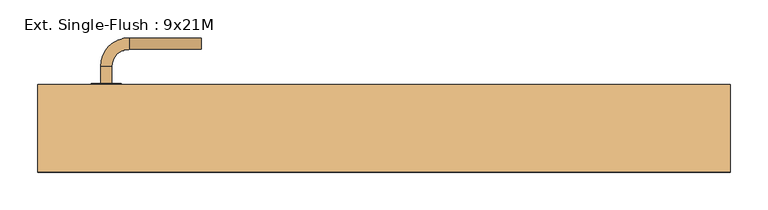
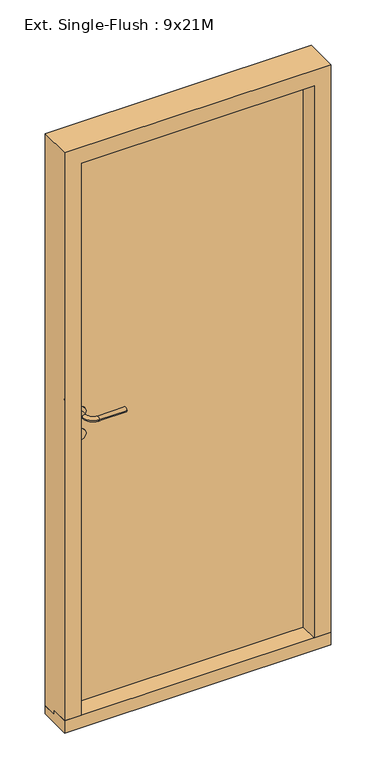
"""IFC4 building model written with IfcOpenShell, lengths in millimetres: door geometry, Ext. Single-Flush : 9x21M."""

from ifc_helpers import new_model, si_unit, point, frame, frame_2d, origin, place, context, project, spatial, polyline, circle_curve, ellipse_curve, trimmed, segment, composite_curve, outline, extrude, faceted_brep, source, transform, mapped, element, save
from ifc_brep_helpers import plane_surface, cylinder_surface, revolved_surface, advanced_brep


def ext_single_flush_9x21m_44480e6f(model_context):
    return source(origin(), model_context, "Body", "SolidModel", [
        extrude(outline(composite_curve([segment(trimmed(circle_curve(frame_2d((1090.0, -366.0)), 20.0), [point((1070.0, -366.0))], [point((1110.0, -366.0))], False, "CARTESIAN"), True, "CONTINUOUS"), segment(trimmed(circle_curve(frame_2d((1090.0, -366.0)), 20.0), [point((1110.0, -366.0))], [point((1070.0, -366.0))], False, "CARTESIAN"), True, "CONTINUOUS")], self_intersect=False)), frame((0.0, 184.0, 0.0), z_axis=(0.0, 1.0, 0.0), x_axis=(0.0, 0.0, 1.0)), (0.0, 0.0, 1.0), 2.0),
        advanced_brep(
        [(-373.5, 186.0, 1090.0), (-358.5, 186.0, 1090.0), (-373.5, 208.5, 1090.0), (-358.5, 208.5, 1090.0), (-336.0, 231.0, 1090.0), (-336.0, 246.0, 1090.0), (-241.0, 246.0, 1090.0), (-241.0, 231.0, 1090.0)],
        [
            (0, 1, circle_curve(frame((-366.0, 186.0, 1090.0), z_axis=(0.0, -1.0, 0.0), x_axis=(1.0, 0.0, 0.0)), 7.5)),
            (1, 0, circle_curve(frame((-366.0, 186.0, 1090.0), z_axis=(0.0, -1.0, 0.0), x_axis=(1.0, 0.0, 0.0)), 7.5)),
            (0, 2),
            (2, 3, circle_curve(frame((-366.0, 208.5, 1090.0), z_axis=(0.0, -1.0, 0.0), x_axis=(1.0, 0.0, 0.0)), 7.5)),
            (3, 1),
            (3, 2, circle_curve(frame((-366.0, 208.5, 1090.0), z_axis=(0.0, -1.0, 0.0), x_axis=(1.0, 0.0, 0.0)), 7.5)),
            (4, 3, circle_curve(frame((-336.0, 208.5, 1090.0), z_axis=(0.0, 0.0, 1.0), x_axis=(-1.0, 0.0, 0.0)), 22.5)),
            (2, 5, circle_curve(frame((-336.0, 208.5, 1090.0), z_axis=(0.0, 0.0, -1.0), x_axis=(-1.0, 0.0, 0.0)), 37.5)),
            (5, 4, circle_curve(frame((-336.0, 238.5, 1090.0), z_axis=(-1.0, 0.0, 0.0), x_axis=(0.0, -1.0, 0.0)), 7.5)),
            (4, 5, circle_curve(frame((-336.0, 238.5, 1090.0), z_axis=(-1.0, 0.0, 0.0), x_axis=(0.0, -1.0, 0.0)), 7.5)),
            (5, 6),
            (6, 7, circle_curve(frame((-241.0, 238.5, 1090.0), z_axis=(-1.0, 0.0, 0.0), x_axis=(0.0, -1.0, 0.0)), 7.5)),
            (7, 4),
            (7, 6, circle_curve(frame((-241.0, 238.5, 1090.0), z_axis=(-1.0, 0.0, 0.0), x_axis=(0.0, -1.0, 0.0)), 7.5)),
        ],
        [
            plane_surface(frame((-366.0, 186.0, 1090.0), z_axis=(0.0, -1.0, 0.0), x_axis=(0.0, 0.0, -1.0))),
            cylinder_surface(frame((-366.0, 186.0, 1090.0), z_axis=(0.0, -1.0, 0.0), x_axis=(1.0, 0.0, 0.0)), 7.5),
            revolved_surface(trimmed(ellipse_curve(frame((-366.0, 208.5, 1090.0), z_axis=(0.0, -1.0, 0.0), x_axis=(1.0, 0.0, 0.0)), 7.5, 7.5), [point((-373.5, 208.5, 1090.0))], [point((-358.5, 208.5, 1090.0))], True, "CARTESIAN"), (-336.0, 208.5, 1090.0), (0.0, 0.0, -1.0)),
            revolved_surface(trimmed(ellipse_curve(frame((-366.0, 208.5, 1090.0), z_axis=(0.0, -1.0, 0.0), x_axis=(1.0, 0.0, 0.0)), 7.5, 7.5), [point((-358.5, 208.5, 1090.0))], [point((-373.5, 208.5, 1090.0))], True, "CARTESIAN"), (-336.0, 208.5, 1090.0), (0.0, 0.0, -1.0)),
            cylinder_surface(frame((-336.0, 238.5, 1090.0), z_axis=(-1.0, 0.0, 0.0), x_axis=(0.0, -1.0, 0.0)), 7.5),
            plane_surface(frame((-241.0, 238.5, 1090.0), z_axis=(1.0, 0.0, 0.0), x_axis=(0.0, 0.0, -1.0))),
        ],
        [
            (0, [[1, 2]]),
            (1, [[-1, 3, 4, 5]]),
            (1, [[-2, -5, 6, -3]]),
            (2, [[7, -4, 8, 9]]),
            (3, [[-8, -6, -7, 10]]),
            (4, [[-9, 11, 12, 13]]),
            (4, [[-10, -13, 14, -11]]),
            (5, [[-14, -12]]),
        ],
    ),
        extrude(outline(composite_curve([segment(trimmed(circle_curve(frame_2d((1010.0, -366.0)), 20.0), [point((990.0, -366.0))], [point((1030.0, -366.0))], False, "CARTESIAN"), True, "CONTINUOUS"), segment(trimmed(circle_curve(frame_2d((1010.0, -366.0)), 20.0), [point((1030.0, -366.0))], [point((990.0, -366.0))], False, "CARTESIAN"), True, "CONTINUOUS")], self_intersect=False), holes=[composite_curve([segment(trimmed(circle_curve(frame_2d((1015.0, -366.0)), 3.0), [point((1012.4019238, -367.5))], [point((1012.4019238, -364.5))], True, "CARTESIAN"), True, "CONTINUOUS"), segment(polyline([(1012.4019238, -364.5), (1000.0, -364.5), (1000.0, -367.5), (1012.4019238, -367.5)]), True, "CONTINUOUS")], self_intersect=False)]), frame((0.0, 184.0, 0.0), z_axis=(0.0, 1.0, 0.0), x_axis=(0.0, 0.0, 1.0)), (0.0, 0.0, 1.0), 2.0),
        extrude(outline(composite_curve([segment(trimmed(circle_curve(frame_2d((1090.0, -366.0)), 20.0), [point((1070.0, -366.0))], [point((1110.0, -366.0))], False, "CARTESIAN"), True, "CONTINUOUS"), segment(trimmed(circle_curve(frame_2d((1090.0, -366.0)), 20.0), [point((1110.0, -366.0))], [point((1070.0, -366.0))], False, "CARTESIAN"), True, "CONTINUOUS")], self_intersect=False)), frame((0.0, 132.0, 0.0), z_axis=(0.0, 1.0, 0.0), x_axis=(0.0, 0.0, 1.0)), (0.0, 0.0, 1.0), 2.0),
        advanced_brep(
        [(-373.5, 132.0, 1090.0), (-358.5, 132.0, 1090.0), (-358.5, 109.5, 1090.0), (-373.5, 109.5, 1090.0), (-336.0, 87.0, 1090.0), (-336.0, 72.0, 1090.0), (-241.0, 87.0, 1090.0), (-241.0, 72.0, 1090.0)],
        [
            (0, 1, circle_curve(frame((-366.0, 132.0, 1090.0), z_axis=(0.0, 1.0, 0.0), x_axis=(1.0, 0.0, 0.0)), 7.5)),
            (1, 0, circle_curve(frame((-366.0, 132.0, 1090.0), z_axis=(0.0, 1.0, 0.0), x_axis=(1.0, 0.0, 0.0)), 7.5)),
            (1, 2),
            (2, 3, circle_curve(frame((-366.0, 109.5, 1090.0), z_axis=(0.0, 1.0, 0.0), x_axis=(1.0, 0.0, 0.0)), 7.5)),
            (3, 0),
            (3, 2, circle_curve(frame((-366.0, 109.5, 1090.0), z_axis=(0.0, 1.0, 0.0), x_axis=(1.0, 0.0, 0.0)), 7.5)),
            (4, 5, circle_curve(frame((-336.0, 79.5, 1090.0), z_axis=(-1.0, 0.0, 0.0), x_axis=(0.0, 1.0, 0.0)), 7.5)),
            (5, 3, circle_curve(frame((-336.0, 109.5, 1090.0), z_axis=(0.0, 0.0, -1.0), x_axis=(-1.0, 0.0, 0.0)), 37.5)),
            (2, 4, circle_curve(frame((-336.0, 109.5, 1090.0), z_axis=(0.0, 0.0, 1.0), x_axis=(-1.0, 0.0, 0.0)), 22.5)),
            (5, 4, circle_curve(frame((-336.0, 79.5, 1090.0), z_axis=(-1.0, 0.0, 0.0), x_axis=(0.0, 1.0, 0.0)), 7.5)),
            (4, 6),
            (6, 7, circle_curve(frame((-241.0, 79.5, 1090.0), z_axis=(-1.0, 0.0, 0.0), x_axis=(0.0, 1.0, 0.0)), 7.5)),
            (7, 5),
            (7, 6, circle_curve(frame((-241.0, 79.5, 1090.0), z_axis=(-1.0, 0.0, 0.0), x_axis=(0.0, 1.0, 0.0)), 7.5)),
        ],
        [
            plane_surface(frame((-366.0, 132.0, 1090.0), z_axis=(0.0, 1.0, 0.0), x_axis=(0.0, 0.0, -1.0))),
            cylinder_surface(frame((-366.0, 132.0, 1090.0), z_axis=(0.0, 1.0, 0.0), x_axis=(1.0, 0.0, 0.0)), 7.5),
            revolved_surface(trimmed(ellipse_curve(frame((-366.0, 109.5, 1090.0), z_axis=(0.0, -1.0, 0.0), x_axis=(1.0, 0.0, 0.0)), 7.5, 7.5), [point((-373.5, 109.5, 1090.0))], [point((-358.5, 109.5, 1090.0))], True, "CARTESIAN"), (-336.0, 109.5, 1090.0), (0.0, 0.0, -1.0)),
            revolved_surface(trimmed(ellipse_curve(frame((-366.0, 109.5, 1090.0), z_axis=(0.0, -1.0, 0.0), x_axis=(1.0, 0.0, 0.0)), 7.5, 7.5), [point((-358.5, 109.5, 1090.0))], [point((-373.5, 109.5, 1090.0))], True, "CARTESIAN"), (-336.0, 109.5, 1090.0), (0.0, 0.0, -1.0)),
            cylinder_surface(frame((-336.0, 79.5, 1090.0), z_axis=(-1.0, 0.0, 0.0), x_axis=(0.0, 1.0, 0.0)), 7.5),
            plane_surface(frame((-241.0, 79.5, 1090.0), z_axis=(1.0, 0.0, 0.0), x_axis=(0.0, 0.0, -1.0))),
        ],
        [
            (0, [[1, 2]]),
            (1, [[3, 4, 5, -2]]),
            (1, [[-5, 6, -3, -1]]),
            (2, [[7, 8, -4, 9]]),
            (3, [[10, -9, -6, -8]]),
            (4, [[11, 12, 13, -7]]),
            (4, [[-13, 14, -11, -10]]),
            (5, [[-12, -14]]),
        ],
    ),
        extrude(outline(composite_curve([segment(trimmed(circle_curve(frame_2d((1010.0, -366.0)), 20.0), [point((990.0, -366.0))], [point((1030.0, -366.0))], False, "CARTESIAN"), True, "CONTINUOUS"), segment(trimmed(circle_curve(frame_2d((1010.0, -366.0)), 20.0), [point((1030.0, -366.0))], [point((990.0, -366.0))], False, "CARTESIAN"), True, "CONTINUOUS")], self_intersect=False), holes=[composite_curve([segment(trimmed(circle_curve(frame_2d((1015.0, -366.0)), 3.0), [point((1012.4019238, -367.5))], [point((1012.4019238, -364.5))], True, "CARTESIAN"), True, "CONTINUOUS"), segment(polyline([(1012.4019238, -364.5), (1000.0, -364.5), (1000.0, -367.5), (1012.4019238, -367.5)]), True, "CONTINUOUS")], self_intersect=False)]), frame((0.0, 132.0, 0.0), z_axis=(0.0, 1.0, 0.0), x_axis=(0.0, 0.0, 1.0)), (0.0, 0.0, 1.0), 2.0),
        extrude(outline(polyline([(-414.0, 184.0), (414.0, 184.0), (414.0, 134.0), (-414.0, 134.0), (-414.0, 184.0)])), frame((0.0, 0.0, 30.0), z_axis=(0.0, 0.0, 1.0), x_axis=(1.0, 0.0, 0.0)), (0.0, 0.0, 1.0), 2028.0),
        faceted_brep([(414.0, 184.0, 2058.0), (-414.0, 184.0, 2058.0), (-414.0, 184.0, 30.0), (-456.0, 184.0, 30.0), (-456.0, 184.0, 2100.0), (456.0, 184.0, 2100.0), (456.0, 184.0, 30.0), (414.0, 184.0, 30.0), (-414.0, 134.0, 2058.0), (-414.0, 134.0, 45.0), (-414.0, 134.0, 30.0), (456.0, 134.0, 30.0), (414.0, 134.0, 30.0), (-456.0, 134.0, 30.0), (-456.0, 69.0, 2100.0), (-456.0, 134.0, 45.0), (-456.0, 69.0, 45.0), (456.0, 69.0, 2100.0), (456.0, 69.0, 45.0), (456.0, 134.0, 45.0), (414.0, 134.0, 2058.0), (414.0, 134.0, 45.0), (-399.0, 69.0, 45.0), (-399.0, 69.0, 2043.0), (399.0, 69.0, 2043.0), (399.0, 69.0, 45.0), (399.0, 134.0, 45.0), (-399.0, 134.0, 45.0), (-399.0, 134.0, 2043.0), (399.0, 134.0, 2043.0)], [[[0, 1, 2, 3, 4, 5, 6, 7]], [[1, 8, 9, 10, 2]], [[11, 12, 7, 6]], [[10, 13, 3, 2]], [[14, 4, 3, 13, 15, 16]], [[5, 17, 18, 19, 11, 6]], [[20, 0, 7, 12, 21]], [[17, 14, 16, 22, 23, 24, 25, 18]], [[21, 19, 18, 25, 26]], [[15, 9, 27, 22, 16]], [[19, 21, 12, 11]], [[9, 15, 13, 10]], [[28, 23, 22, 27]], [[24, 29, 26, 25]], [[29, 28, 27, 9, 8, 20, 21, 26]], [[5, 4, 14, 17]], [[24, 23, 28, 29]], [[1, 0, 20, 8]]]),
        extrude(outline(polyline([(184.0, 30.0), (184.0, 0.0), (69.0, 0.0), (69.0, 45.0), (134.0, 45.0), (134.0, 30.0), (184.0, 30.0)])), frame((-456.0, 0.0, 0.0), z_axis=(1.0, 0.0, 0.0), x_axis=(0.0, 1.0, 0.0)), (0.0, 0.0, 1.0), 912.0),
    ])


if __name__ == "__main__":
    model = new_model("IFC4")
    model_context = context("Model", 3, world=origin())
    ifc_project = project(units=[si_unit("LENGTHUNIT", "METRE", prefix="MILLI")], contexts=[model_context])
    site = spatial("IfcSite", under=ifc_project)
    building = spatial("IfcBuilding", under=site)
    placement = place(None, origin())
    ext_single_flush_9x21m_shape = ext_single_flush_9x21m_44480e6f(model_context)
    element("IfcDoor", 1, ObjectType="Ext. Single-Flush : 9x21M", at=placement, inside=building, context=model_context, shape_type="MappedRepresentation", body=[
        mapped(ext_single_flush_9x21m_shape, transform((0.0, 0.0, 0.0), x_axis=(1.0, 0.0, 0.0), y_axis=(0.0, 1.0, 0.0), z_axis=(0.0, 0.0, 1.0))),
    ])
    save(model, "model.ifc")

# Revit data of these elements
# Project information
#   Client Name = "Test Project"
#   Project Address = "Enter address here"
#   Project Number = "Number"
#   Current Version = "0.0.0"
#   SR Document GUID = "3eb9317e-835d-4f79-8926-4d15b96bc824"
# Type "Ext. Single-Flush : 9x21M"
#   Type Mark = "51"
#   Sound Rating = ""
#   Opening Side [instance default] = ""
#   Hinge Side [instance default] = ""
#   Creator Organization [instance default] = "© Danish Educational Content"
#   Creator Name [instance default] = "© Erik Falck Jørgensen"
#   Creator Build [instance default] = "2017.0301.0"
#   Analytic Construction = "<None>"
#   length#6 = -50 mm
#   length#5 = 912 mm
#   length#4 = 120 mm
#   length#3 = 30 mm
#   length#2 = 57 mm
#   length#1 = 0 mm
#   Thickness = 50 mm
#   Seal Width = 12 mm
#   Rough Width = 912 mm
#   Rough Height = 2100 mm
#   Rebate Depth = 50 mm
#   Rabbet Width = 15 mm
#   Rabbet Depth = 50 mm
#   Height = 2088 mm
#   Width = 888 mm
#   Handle From Side = 90 mm
#   Handle From Bottom = 1090 mm
#   Exterior Direction [instance default] = 0.00°
#   Case Width = 45 mm
#   Case Depth = 115 mm
#   Threshold = yes
#   Sealing = no
#   Hinging = yes
#   Wall Closure = 1
#   Function = 1
#   Panel = none
#   Handle Finish = none
#   Handle = element 507533
#   Embrasure Interior = none
#   Embrasure Exterior = none
#   Case/Transom = none
#   Assembly Code = ""
# Element 1 (IfcDoor, "Ext. Single-Flush : 9x21M")
#   Materials on its faces: "Stainless Steel, Polished", "Default Frame/Mullion (Interior/Exterior)", "Default Door Panel (Exterior/Interior)"
# Materials
#   "Stainless Steel, Polished": class "Metal", colour RGB 180 180 180, transparency 0, Description = "Rustfri stål, poleret", Cost = 0
#   "Default Frame/Mullion (Interior/Exterior)": class "Generic", colour RGB 205 205 205, transparency 0, Description = "Udefineret karm/ramme materiale", Cost = 0
#   "Default Door Panel (Exterior/Interior)": class "Generic", colour RGB 205 205 205, transparency 0, Description = "Udefineret dørplade materiale", Cost = 0
